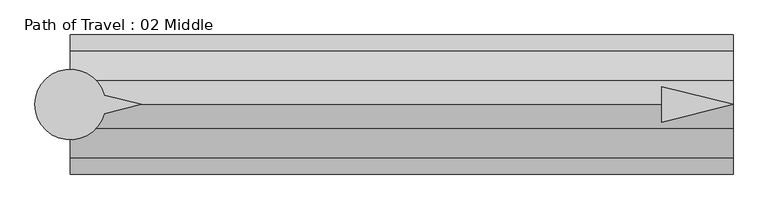
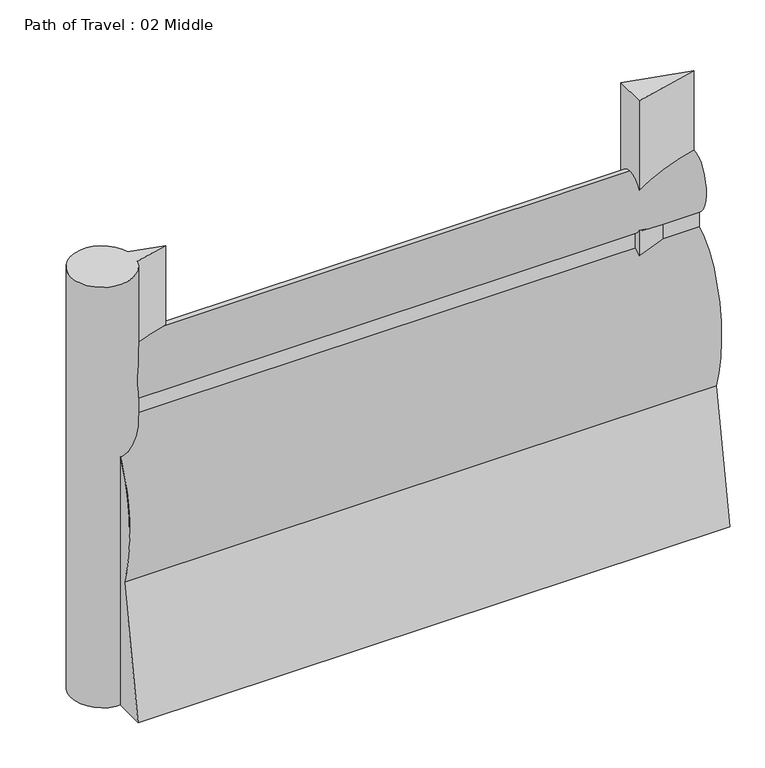
"""IFC4 building model written with IfcOpenShell, lengths in millimetres: proxy geometry, Path of Travel : 02 Middle."""

from ifc_helpers import new_model, si_unit, point, frame, frame_2d, origin, origin_with_axes, place, context, project, spatial, polyline, circle_curve, ellipse_curve, trimmed, segment, composite_curve, outline, extrude, source, transform, mapped, element, save
from ifc_brep_helpers import plane_surface, extruded_surface, advanced_brep


def path_of_travel_02_middle_bc2c9401(model_context):
    return source(origin(), model_context, "Body", "SolidModel", [
        advanced_brep(
        [(227.5554837, 0.0, 1727.2), (227.5554837, 42.9018657, 1436.6534209), (227.5554837, 42.9018657, 1363.4763406), (227.5554837, 184.1186263, 643.4144547), (227.5554837, 297.5699544, 0.0), (227.5554837, 145.6574193, 0.0), (227.5554837, 0.0, 584.2), (227.5554837, -145.6574193, 0.0), (227.5554837, -297.5699544, 0.0), (227.5554837, -184.1186263, 643.4144547), (227.5554837, -42.9018657, 1363.4763406), (227.5554837, -42.9018657, 1436.6534209), (3064.1585306, 0.0, 1727.2), (3064.1585306, -42.9018657, 1436.6534209), (3064.1585306, -42.9018657, 1363.4763406), (3064.1585306, -184.1186263, 643.4144547), (3064.1585306, -297.5699544, 0.0), (3064.1585306, -145.6574193, 0.0), (3064.1585306, 0.0, 584.2), (3064.1585306, 145.6574193, 0.0), (3064.1585306, 297.5699544, 0.0), (3064.1585306, 184.1186263, 643.4144547), (3064.1585306, 42.9018657, 1363.4763406), (3064.1585306, 42.9018657, 1436.6534209)],
        [
            (0, 1, ellipse_curve(frame((227.5554837, 0.0, 1574.8), z_axis=(-1.0, 0.0, 0.0), x_axis=(0.0, 0.0, 1.0)), 152.4, 101.6)),
            (1, 2),
            (2, 3, ellipse_curve(frame((227.5554837, 0.0, 914.4), z_axis=(-1.0, 0.0, 0.0), x_axis=(0.0, 0.0, -1.0)), 457.2, 228.6)),
            (3, 4),
            (4, 5),
            (5, 6),
            (6, 7),
            (7, 8),
            (8, 9),
            (9, 10, ellipse_curve(frame((227.5554837, 0.0, 914.4), z_axis=(-1.0, 0.0, 0.0), x_axis=(0.0, 0.0, -1.0)), 457.2, 228.6)),
            (10, 11),
            (11, 0, ellipse_curve(frame((227.5554837, 0.0, 1574.8), z_axis=(-1.0, 0.0, 0.0), x_axis=(0.0, 0.0, 1.0)), 152.4, 101.6)),
            (12, 13, ellipse_curve(frame((3064.1585306, 0.0, 1574.8), z_axis=(1.0, 0.0, 0.0), x_axis=(0.0, 0.0, 1.0)), 152.4, 101.6)),
            (13, 14),
            (14, 15, ellipse_curve(frame((3064.1585306, 0.0, 914.4), z_axis=(1.0, 0.0, 0.0), x_axis=(0.0, 0.0, -1.0)), 457.2, 228.6)),
            (15, 16),
            (16, 17),
            (17, 18),
            (18, 19),
            (19, 20),
            (20, 21),
            (21, 22, ellipse_curve(frame((3064.1585306, 0.0, 914.4), z_axis=(1.0, 0.0, 0.0), x_axis=(0.0, 0.0, -1.0)), 457.2, 228.6)),
            (22, 23),
            (23, 12, ellipse_curve(frame((3064.1585306, 0.0, 1574.8), z_axis=(1.0, 0.0, 0.0), x_axis=(0.0, 0.0, 1.0)), 152.4, 101.6)),
            (0, 12),
            (23, 1),
            (22, 2),
            (21, 3),
            (20, 4),
            (19, 5),
            (18, 6),
            (17, 7),
            (16, 8),
            (15, 9),
            (14, 10),
            (13, 11),
        ],
        [
            plane_surface(frame((227.5554837, 0.0, 0.0), z_axis=(-1.0, 0.0, 0.0), x_axis=(0.0, 0.0, 1.0))),
            plane_surface(frame((3064.1585306, 0.0, 0.0), z_axis=(1.0, 0.0, 0.0), x_axis=(0.0, 0.0, 1.0))),
            extruded_surface(trimmed(ellipse_curve(frame((3064.1585306, 0.0, 1574.8), z_axis=(-1.0, 0.0, 0.0), x_axis=(0.0, 0.0, 1.0)), 152.4, 101.6), [point((3064.1585306, 0.0, 1727.2))], [point((3064.1585306, 42.9018657, 1436.6534209))], True, "CARTESIAN"), (-2836.6030469, 0.0, 0.0), 2836.6030469),
            plane_surface(frame((227.5554837, 42.9018657, 1436.6534209), z_axis=(0.0, 1.0, 0.0), x_axis=(1.0, 0.0, 0.0))),
            extruded_surface(trimmed(ellipse_curve(frame((3064.1585306, 0.0, 914.4), z_axis=(-1.0, 0.0, 0.0), x_axis=(0.0, 0.0, -1.0)), 457.2, 228.6), [point((3064.1585306, 42.9018657, 1363.4763406))], [point((3064.1585306, 184.1186263, 643.4144547))], True, "CARTESIAN"), (-2836.6030469, 0.0, 0.0), 2836.6030469),
            plane_surface(frame((227.5554837, 184.1186263, 643.4144547), z_axis=(0.0, 0.9848077530122078, 0.1736481776669322), x_axis=(1.0, 0.0, 0.0))),
            plane_surface(frame((227.5554837, 297.5699544, 0.0), z_axis=(0.0, 0.0, -1.0), x_axis=(1.0, 0.0, 0.0))),
            plane_surface(frame((227.5554837, 145.6574193, 0.0), z_axis=(0.0, -0.9702957262760199, -0.2419218955995739), x_axis=(1.0, 0.0, 0.0))),
            plane_surface(frame((227.5554837, 0.0, 584.2), z_axis=(0.0, 0.9702957262759961, -0.24192189559966923), x_axis=(1.0, 0.0, 0.0))),
            plane_surface(frame((227.5554837, -145.6574193, 0.0), z_axis=(0.0, 0.0, -1.0), x_axis=(1.0, 0.0, 0.0))),
            plane_surface(frame((227.5554837, -297.5699544, 0.0), z_axis=(0.0, -0.984807753012208, 0.17364817766693066), x_axis=(1.0, 0.0, 0.0))),
            extruded_surface(trimmed(ellipse_curve(frame((3064.1585306, 0.0, 914.4), z_axis=(-1.0, 0.0, 0.0), x_axis=(0.0, 0.0, -1.0)), 457.2, 228.6), [point((3064.1585306, -184.1186263, 643.4144547))], [point((3064.1585306, -42.9018657, 1363.4763406))], True, "CARTESIAN"), (-2836.6030469, 0.0, 0.0), 2836.6030469),
            plane_surface(frame((227.5554837, -42.9018657, 1363.4763406), z_axis=(0.0, -1.0, 0.0), x_axis=(1.0, 0.0, 0.0))),
            extruded_surface(trimmed(ellipse_curve(frame((3064.1585306, 0.0, 1574.8), z_axis=(-1.0, 0.0, 0.0), x_axis=(0.0, 0.0, 1.0)), 152.4, 101.6), [point((3064.1585306, -42.9018657, 1436.6534209))], [point((3064.1585306, 0.0, 1727.2))], True, "CARTESIAN"), (-2836.6030469, 0.0, 0.0), 2836.6030469),
        ],
        [
            (0, [[1, 2, 3, 4, 5, 6, 7, 8, 9, 10, 11, 12]]),
            (1, [[13, 14, 15, 16, 17, 18, 19, 20, 21, 22, 23, 24]]),
            (2, [[-1, 25, -24, 26]]),
            (3, [[-2, -26, -23, 27]]),
            (4, [[-3, -27, -22, 28]]),
            (5, [[-4, -28, -21, 29]]),
            (6, [[-5, -29, -20, 30]]),
            (7, [[-6, -30, -19, 31]]),
            (8, [[-7, -31, -18, 32]]),
            (9, [[-8, -32, -17, 33]]),
            (10, [[-9, -33, -16, 34]]),
            (11, [[-10, -34, -15, 35]]),
            (12, [[-11, -35, -14, 36]]),
            (13, [[-12, -36, -13, -25]]),
        ],
    ),
        extrude(outline(polyline([(2758.1533841, 76.2006338), (3064.1585306, 0.0), (2758.1533841, -76.2006338), (2758.1533841, 76.2006338)])), origin_with_axes(), (0.0, 0.0, 1.0), 2129.5973753),
        extrude(outline(composite_curve([segment(polyline([(372.7837828, 39.4440225), (531.182385, 0.0), (372.7837828, -39.4440225)]), True, "CONTINUOUS"), segment(trimmed(circle_curve(frame_2d((227.2200886, 0.0)), 150.8131956), [point((372.7837828, -39.4440225))], [point((372.7837828, 39.4440225))], False, "CARTESIAN"), True, "CONTINUOUS")], self_intersect=False)), origin_with_axes(), (0.0, 0.0, 1.0), 2129.5973753),
    ])


if __name__ == "__main__":
    model = new_model("IFC4")
    model_context = context("Model", 3, world=origin())
    ifc_project = project(units=[si_unit("LENGTHUNIT", "METRE", prefix="MILLI")], contexts=[model_context])
    site = spatial("IfcSite", under=ifc_project)
    building = spatial("IfcBuilding", under=site)
    placement = place(None, origin())
    path_of_travel_02_middle_shape = path_of_travel_02_middle_bc2c9401(model_context)
    element("IfcBuildingElementProxy", 1, Name="Path of Travel : 02 Middle", ObjectType="Path of Travel : 02 Middle", at=placement, inside=building, context=model_context, shape_type="MappedRepresentation", body=[
        mapped(path_of_travel_02_middle_shape, transform((0.0, 0.0, 0.0), x_axis=(1.0, 0.0, 0.0), y_axis=(0.0, 1.0, 0.0), z_axis=(0.0, 0.0, 1.0))),
    ])
    save(model, "model.ifc")

# Revit data of these elements
# Type "Path of Travel : 02 Middle"
#   Path of Egress [instance default] = 4' - 0"
#   built-in parameter 1001306 [instance default] = 4 (stored number, unit not read)
#   Dot at Start = no
#   Arrow in Middle = yes
#   Arrow at End = no
#   Egress Path = none
# Element 1 (IfcBuildingElementProxy, "Path of Travel : 02 Middle")
#   Path of Egress = 9' - 3.67729"
#   built-in parameter 1001306 = 9.30644 (stored number, unit not read)
